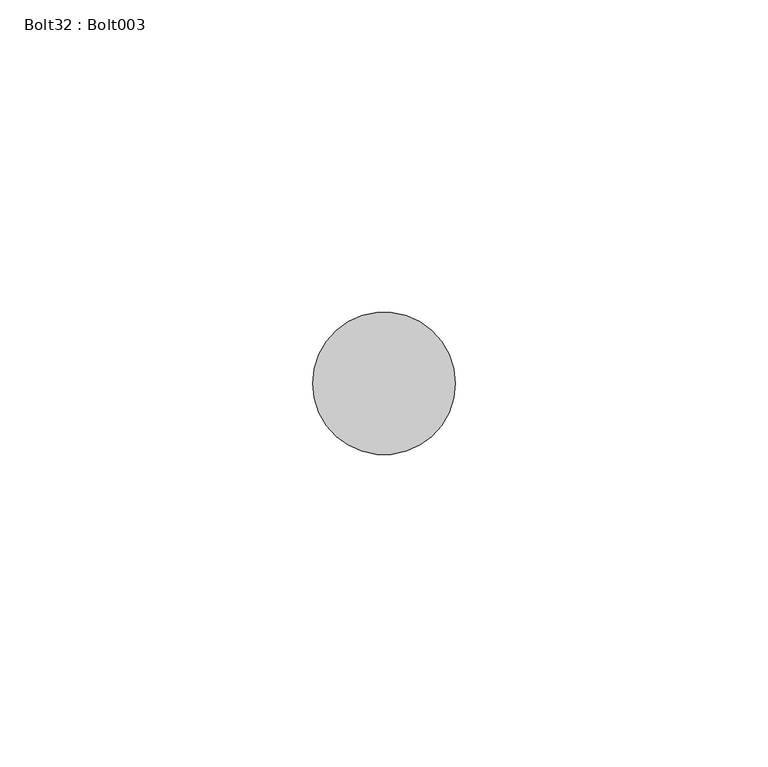
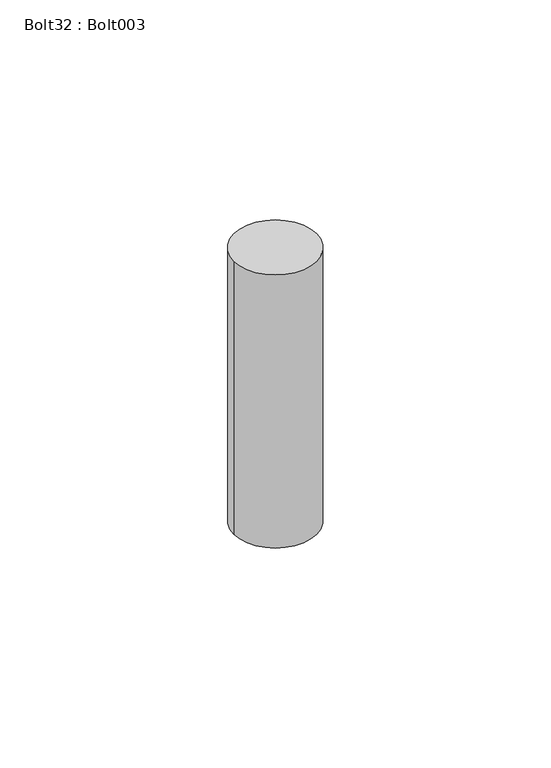
"""IFC4 building model written with IfcOpenShell, lengths in millimetres: proxy geometry, Bolt32 : Bolt003."""

from ifc_helpers import new_model, si_unit, point, frame, frame_2d, origin, place, context, project, spatial, circle_curve, trimmed, segment, composite_curve, outline, extrude, source, transform, mapped, element, save


def bolt32_bolt003_c7632ded(model_context):
    return source(origin(), model_context, "Body", "SweptSolid", [
        extrude(outline(composite_curve([segment(trimmed(circle_curve(frame_2d((5062.3346014, 1998.1882072)), 11.4045168), [point((5073.7391183, 1998.1882072))], [point((5050.9300846, 1998.1882072))], False, "CARTESIAN"), True, "CONTINUOUS"), segment(trimmed(circle_curve(frame_2d((5062.3346014, 1998.1882072)), 11.4045168), [point((5050.9300846, 1998.1882072))], [point((5073.7391183, 1998.1882072))], False, "CARTESIAN"), True, "CONTINUOUS")], self_intersect=False)), frame((0.0, 0.0, 36645.5959962), z_axis=(0.0, 0.0, 1.0), x_axis=(1.0, 0.0, 0.0)), (0.0, 0.0, 1.0), 79.375),
    ])


if __name__ == "__main__":
    model = new_model("IFC4")
    model_context = context("Model", 3, world=origin())
    ifc_project = project(units=[si_unit("LENGTHUNIT", "METRE", prefix="MILLI")], contexts=[model_context])
    site = spatial("IfcSite", under=ifc_project)
    building = spatial("IfcBuilding", under=site)
    placement = place(None, origin())
    bolt32_bolt003_shape = bolt32_bolt003_c7632ded(model_context)
    element("IfcBuildingElementProxy", 1, Name="Bolt32 : Bolt003", ObjectType="Bolt32 : Bolt003", at=placement, inside=building, context=model_context, shape_type="MappedRepresentation", body=[
        mapped(bolt32_bolt003_shape, transform((0.0, 0.0, 0.0), x_axis=(1.0, 0.0, 0.0), y_axis=(0.0, 1.0, 0.0), z_axis=(0.0, 0.0, 1.0))),
    ])
    save(model, "model.ifc")

# Revit data of these elements
# Type "Bolt32 : Bolt003"
#   NameOverride = "Bolt003"
# Element 1 (IfcBuildingElementProxy, "Bolt32 : Bolt003")
#   Materials on its faces: "STEEL ANGLE AND ANCHOR BOLT (SEE STRUCT. DWGS)"
# Materials
#   "STEEL ANGLE AND ANCHOR BOLT (SEE STRUCT. DWGS)": class "Unassigned", colour RGB 128 128 128, transparency 0, Cost = 0
